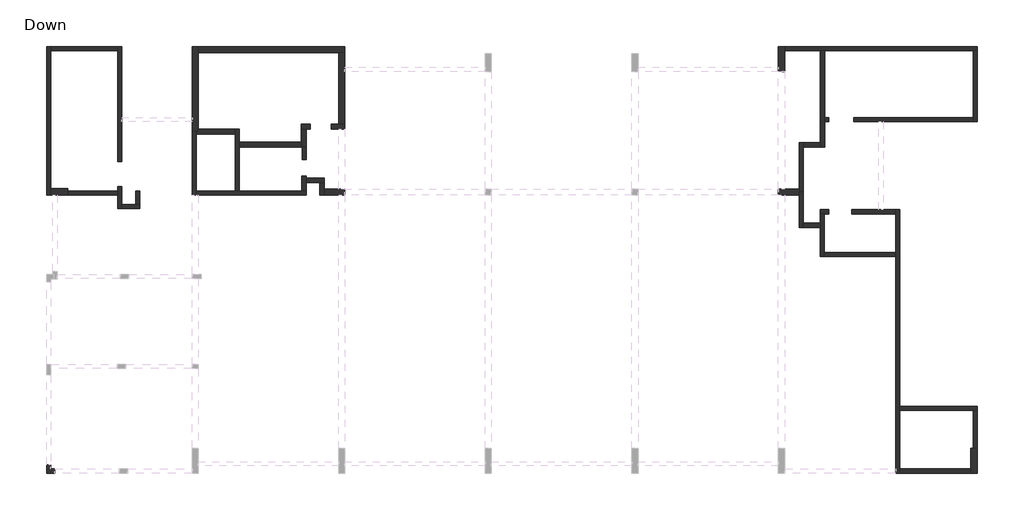
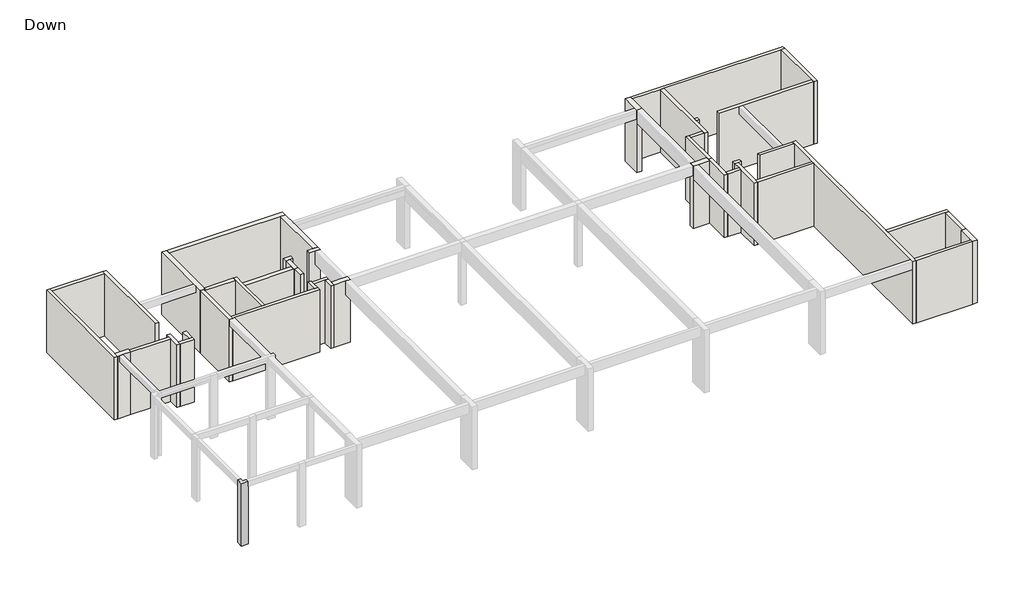
# One storey, part 1 of 2: 44 walls, 1 column.
"""IFC4 building model written with IfcOpenShell, lengths in millimetres."""

from ifc_helpers import new_model, si_unit, origin, origin_with_axes, place, context, project, spatial, polyline, outline, extrude, faceted_brep, element, save

model = new_model("IFC4")

# Units and contexts
model_context = context("Model", 3, world=origin())
ifc_project = project(units=[si_unit("LENGTHUNIT", "METRE", prefix="MILLI")], contexts=[model_context])

# Site, building, storey
site = spatial("IfcSite", under=ifc_project)
building = spatial("IfcBuilding", under=site)
storey = spatial("IfcBuildingStorey", under=building, Name="Down", Elevation=0.0)

# Column
placement = place(None, origin())
element("IfcColumn", 1, ObjectType="L Column : 40/40/20/20", at=placement, inside=storey, context=model_context, shape_type="Brep", body=[
    faceted_brep([(-20892.8250626, 4006.6682295, 0.0), (-20892.8250626, 4406.6682295, 0.0), (-20692.8250626, 4406.6682295, 0.0), (-20692.8250626, 4206.6682295, 0.0), (-20492.8250626, 4206.6682295, 0.0), (-20492.8250626, 4006.6682295, 0.0), (-20892.8250626, 4006.6682295, 4000.0), (-20892.8250626, 4406.6682295, 4000.0), (-20692.8250626, 4406.6682295, 4000.0), (-20692.8250626, 4206.6682295, 4000.0), (-20690.7944112, 4206.6682295, 4000.0), (-20492.8250626, 4206.6682295, 4000.0), (-20492.8250626, 4006.6682295, 4000.0)], [[[0, 1, 2, 3, 4, 5]], [[6, 7, 1, 0]], [[7, 8, 2, 1]], [[8, 9, 3, 2]], [[9, 10, 11, 4, 3]], [[11, 12, 5, 4]], [[12, 6, 0, 5]], [[6, 12, 11, 10, 9, 8, 7]]]),
])

# Walls
element("IfcWall", 2, ObjectType="20", at=placement, inside=storey, context=model_context, shape_type="Brep", body=[
    faceted_brep([(-20890.7944112, 24404.7142065, 0.0), (-20890.7944112, 17304.7716778, 0.0), (-20890.7944112, 17304.7716778, 4000.0), (-20890.7944112, 24404.7142065, 4000.0), (-20690.7944112, 24404.7142065, 0.0), (-20690.7944112, 24404.7142065, 4000.0), (-20690.7944112, 24204.7142065, 4000.0), (-20690.7944112, 19305.3655475, 4000.0), (-20690.7944112, 17605.3655475, 4000.0), (-20690.7944112, 17305.3655475, 4000.0), (-20690.7944112, 17304.7716778, 4000.0), (-20690.7944112, 17304.7716778, 0.0), (-20690.7944112, 17305.3655475, 0.0), (-20690.7944112, 17605.3655475, 0.0), (-20690.7944112, 24204.7142065, 0.0)], [[[0, 1, 2, 3]], [[4, 5, 6, 7, 8, 9, 10, 11, 12, 13, 14]], [[1, 0, 4, 14, 13, 12, 11]], [[2, 1, 11, 10]], [[3, 2, 10, 9, 8, 7, 6, 5]], [[0, 3, 5, 4]]]),
])
element("IfcWall", 3, ObjectType="20", at=placement, inside=storey, context=model_context, shape_type="Brep", body=[
    faceted_brep([(-19891.6373231, 17304.7716778, 0.0), (-17492.1354074, 17304.7716778, 0.0), (-17492.1354074, 17304.7716778, 3790.0), (-17492.1354074, 17304.7716778, 4000.0), (-19891.6373231, 17304.7716778, 4000.0), (-19891.6373231, 17304.7716778, 3790.0), (-19891.6373231, 17504.7716778, 0.0), (-19891.6373231, 17504.7716778, 3790.0), (-19891.6373231, 17504.7716778, 4000.0), (-17492.1354074, 17504.7716778, 4000.0), (-17492.1354074, 17504.7716778, 3790.0), (-17492.1354074, 17504.7716778, 0.0), (-19891.6373231, 17305.3655475, 0.0), (-19891.6373231, 17305.3655475, 4000.0)], [[[0, 1, 2, 3, 4, 5]], [[6, 7, 8, 9, 10, 11]], [[1, 0, 12, 6, 11]], [[4, 3, 9, 8, 13]], [[0, 5, 4, 13, 8, 7, 6, 12]], [[3, 2, 1, 11, 10, 9]]]),
])
element("IfcWall", 4, ObjectType="20", at=placement, inside=storey, context=model_context, shape_type="Brep", body=[
    faceted_brep([(-17492.1354074, 17706.9747429, 0.0), (-17492.1354074, 17504.7716778, 0.0), (-17492.1354074, 17304.7716778, 0.0), (-17492.1354074, 16652.7793406, 0.0), (-17492.1354074, 16652.7793406, 3790.0), (-17492.1354074, 16652.7793406, 4000.0), (-17492.1354074, 17304.7716778, 4000.0), (-17492.1354074, 17504.7716778, 4000.0), (-17492.1354074, 17706.9747429, 4000.0), (-17492.1354074, 17706.9747429, 3790.0), (-17292.1354074, 17706.9747429, 0.0), (-17292.1354074, 17706.9747429, 3790.0), (-17292.1354074, 17706.9747429, 4000.0), (-17292.1354074, 16852.7793406, 4000.0), (-17292.1354074, 16652.7793406, 4000.0), (-17292.1354074, 16652.7793406, 0.0), (-17292.1354074, 16852.7793406, 0.0)], [[[0, 1, 2, 3, 4, 5, 6, 7, 8, 9]], [[10, 11, 12, 13, 14, 15, 16]], [[3, 2, 1, 0, 10, 16, 15]], [[8, 7, 6, 5, 14, 13, 12]], [[0, 9, 8, 12, 11, 10]], [[5, 4, 3, 15, 14]]]),
])
element("IfcWall", 5, ObjectType="20", at=placement, inside=storey, context=model_context, shape_type="Brep", body=[
    faceted_brep([(-17292.1354074, 18905.1165054, 0.0), (-17292.1354074, 24404.7142065, 0.0), (-17292.1354074, 24404.7142065, 4000.0), (-17292.1354074, 20806.0552027, 4000.0), (-17292.1354074, 18905.1165054, 4000.0), (-17292.1354074, 18905.1165054, 3790.0), (-17492.1354074, 18905.1165054, 0.0), (-17492.1354074, 18905.1165054, 3790.0), (-17492.1354074, 18905.1165054, 4000.0), (-17492.1354074, 19305.3655475, 4000.0), (-17492.1354074, 24204.7142065, 4000.0), (-17492.1354074, 24404.7142065, 4000.0), (-17492.1354074, 24404.7142065, 0.0), (-17492.1354074, 24204.7142065, 0.0)], [[[0, 1, 2, 3, 4, 5]], [[6, 7, 8, 9, 10, 11, 12, 13]], [[1, 0, 6, 13, 12]], [[4, 3, 2, 11, 10, 9, 8]], [[0, 5, 4, 8, 7, 6]], [[2, 1, 12, 11]]]),
])
element("IfcWall", 6, ObjectType="20", at=placement, inside=storey, context=model_context, shape_type="SweptSolid", body=[
    extrude(outline(polyline([(-20690.7944112, 24404.7142065), (-17492.1354074, 24404.7142065), (-17492.1354074, 24204.7142065), (-20690.7944112, 24204.7142065), (-20690.7944112, 24404.7142065)])), origin_with_axes(), (0.0, 0.0, 1.0), 4000.0),
])
element("IfcWall", 7, ObjectType="20", at=placement, inside=storey, context=model_context, shape_type="Brep", body=[
    faceted_brep([(-17292.1354074, 16652.7793406, 0.0), (-16441.1583959, 16652.7793406, 0.0), (-16441.1583959, 16652.7793406, 3790.0), (-16441.1583959, 16652.7793406, 4000.0), (-17292.1354074, 16652.7793406, 4000.0), (-17292.1354074, 16852.7793406, 0.0), (-17292.1354074, 16852.7793406, 3790.0), (-17292.1354074, 16852.7793406, 4000.0), (-16641.1583959, 16852.7793406, 4000.0), (-16441.1583959, 16852.7793406, 4000.0), (-16441.1583959, 16852.7793406, 0.0), (-16641.1583959, 16852.7793406, 0.0)], [[[0, 1, 2, 3, 4]], [[5, 6, 7, 8, 9, 10, 11]], [[1, 0, 5, 11, 10]], [[4, 3, 9, 8, 7]], [[0, 4, 7, 6, 5]], [[3, 2, 1, 10, 9]]]),
])
element("IfcWall", 8, ObjectType="20", at=placement, inside=storey, context=model_context, shape_type="Brep", body=[
    faceted_brep([(-16441.1583959, 16852.7793406, 0.0), (-16441.1583959, 17503.7563521, 0.0), (-16441.1583959, 17503.7563521, 3790.0), (-16441.1583959, 17503.7563521, 4000.0), (-16441.1583959, 16852.7793406, 4000.0), (-16641.1583959, 16852.7793406, 0.0), (-16641.1583959, 16852.7793406, 3790.0), (-16641.1583959, 16852.7793406, 4000.0), (-16641.1583959, 17503.7563521, 4000.0), (-16641.1583959, 17503.7563521, 3790.0), (-16641.1583959, 17503.7563521, 0.0)], [[[0, 1, 2, 3, 4]], [[5, 6, 7, 8, 9, 10]], [[1, 0, 5, 10]], [[3, 2, 1, 10, 9, 8]], [[4, 3, 8, 7]], [[0, 4, 7, 6, 5]]]),
])
element("IfcWall", 9, ObjectType="20", at=placement, inside=storey, context=model_context, shape_type="Brep", body=[
    faceted_brep([(-11890.9285108, 20459.7142065, 0.0), (-11890.9285108, 20209.7142065, 0.0), (-11890.9285108, 17504.7716778, 0.0), (-11890.9285108, 17504.7716778, 4000.0), (-11890.9285108, 20209.7142065, 4000.0), (-11890.9285108, 20459.7142065, 4000.0), (-11690.9285108, 20459.7142065, 0.0), (-11690.9285108, 20459.7142065, 3790.0), (-11690.9285108, 20459.7142065, 4000.0), (-11690.9285108, 19844.6567352, 4000.0), (-11690.9285108, 19594.6567352, 4000.0), (-11690.9285108, 17504.7716778, 4000.0), (-11690.9285108, 17504.7716778, 3790.0), (-11690.9285108, 17504.7716778, 0.0), (-11690.9285108, 19594.6567352, 0.0), (-11690.9285108, 19844.6567352, 0.0)], [[[0, 1, 2, 3, 4, 5]], [[6, 7, 8, 9, 10, 11, 12, 13, 14, 15]], [[2, 1, 0, 6, 15, 14, 13]], [[5, 4, 3, 11, 10, 9, 8]], [[3, 2, 13, 12, 11]], [[0, 5, 8, 7, 6]]]),
])
element("IfcWall", 10, ObjectType="20", at=placement, inside=storey, context=model_context, shape_type="Brep", body=[
    faceted_brep([(-13743.2656756, 17304.7716778, 0.0), (-8494.4725721, 17304.7716778, 0.0), (-8494.4725721, 17304.7716778, 3790.0), (-8494.4725721, 17304.7716778, 4000.0), (-13643.2656756, 17304.7716778, 4000.0), (-13743.2656756, 17304.7716778, 4000.0), (-13743.2656756, 17504.7716778, 0.0), (-13743.2656756, 17504.7716778, 4000.0), (-11890.9285108, 17504.7716778, 4000.0), (-11690.9285108, 17504.7716778, 4000.0), (-8694.4725721, 17504.7716778, 4000.0), (-8494.4725721, 17504.7716778, 4000.0), (-8494.4725721, 17504.7716778, 0.0), (-8694.4725721, 17504.7716778, 0.0), (-11690.9285108, 17504.7716778, 0.0), (-11890.9285108, 17504.7716778, 0.0)], [[[0, 1, 2, 3, 4, 5]], [[6, 7, 8, 9, 10, 11, 12, 13, 14, 15]], [[1, 0, 6, 15, 14, 13, 12]], [[5, 4, 3, 11, 10, 9, 8, 7]], [[3, 2, 1, 12, 11]], [[0, 5, 7, 6]]]),
])
element("IfcWall", 11, ObjectType="20", at=placement, inside=storey, context=model_context, shape_type="Brep", body=[
    faceted_brep([(-8494.4725721, 17504.7716778, 0.0), (-8494.4725721, 17905.9594172, 0.0), (-8494.4725721, 18105.9594172, 0.0), (-8494.4725721, 18206.553287, 0.0), (-8494.4725721, 18206.553287, 3790.0), (-8494.4725721, 18206.553287, 4000.0), (-8494.4725721, 18105.9594172, 4000.0), (-8494.4725721, 17905.9594172, 4000.0), (-8494.4725721, 17504.7716778, 4000.0), (-8694.4725721, 17504.7716778, 0.0), (-8694.4725721, 17504.7716778, 3790.0), (-8694.4725721, 17504.7716778, 4000.0), (-8694.4725721, 18206.553287, 4000.0), (-8694.4725721, 18206.553287, 3790.0), (-8694.4725721, 18206.553287, 0.0)], [[[0, 1, 2, 3, 4, 5, 6, 7, 8]], [[9, 10, 11, 12, 13, 14]], [[3, 2, 1, 0, 9, 14]], [[5, 4, 3, 14, 13, 12]], [[8, 7, 6, 5, 12, 11]], [[0, 8, 11, 10, 9]]]),
])
element("IfcWall", 12, ObjectType="20", at=placement, inside=storey, context=model_context, shape_type="Brep", body=[
    faceted_brep([(-8485.7944112, 19006.7257008, 0.0), (-8485.7944112, 19594.6567352, 0.0), (-8485.7944112, 19594.6567352, 4000.0), (-8485.7944112, 19006.7257008, 4000.0), (-8485.7944112, 19006.7257008, 3790.0), (-8685.7944112, 19006.7257008, 0.0), (-8685.7944112, 19006.7257008, 3790.0), (-8685.7944112, 19006.7257008, 4000.0), (-8685.7944112, 19594.6567352, 4000.0), (-8685.7944112, 19594.6567352, 3790.0), (-8685.7944112, 19594.6567352, 0.0)], [[[0, 1, 2, 3, 4]], [[5, 6, 7, 8, 9, 10]], [[1, 0, 5, 10]], [[3, 2, 8, 7]], [[0, 4, 3, 7, 6, 5]], [[2, 1, 10, 9, 8]]]),
])
element("IfcWall", 13, ObjectType="20", at=placement, inside=storey, context=model_context, shape_type="Brep", body=[
    faceted_brep([(-13943.2656756, 20334.7142065, 0.0), (-13943.2656756, 17304.7716778, 0.0), (-13943.2656756, 17304.7716778, 3600.0), (-13943.2656756, 17304.7716778, 4000.0), (-13943.2656756, 20334.7142065, 4000.0), (-13743.2656756, 20334.7142065, 0.0), (-13743.2656756, 20334.7142065, 4000.0), (-13743.2656756, 20209.7142065, 4000.0), (-13743.2656756, 17504.7716778, 4000.0), (-13743.2656756, 17304.7716778, 4000.0), (-13743.2656756, 17304.7716778, 0.0), (-13743.2656756, 17504.7716778, 0.0), (-13743.2656756, 20209.7142065, 0.0)], [[[0, 1, 2, 3, 4]], [[5, 6, 7, 8, 9, 10, 11, 12]], [[1, 0, 5, 12, 11, 10]], [[4, 3, 9, 8, 7, 6]], [[0, 4, 6, 5]], [[3, 2, 1, 10, 9]]]),
])
element("IfcWall", 14, ObjectType="20", at=placement, inside=storey, context=model_context, shape_type="Brep", body=[
    faceted_brep([(-8494.4725721, 17905.9594172, 0.0), (-7834.4725721, 17905.9594172, 0.0), (-7634.4725721, 17905.9594172, 0.0), (-7634.4725721, 17905.9594172, 4000.0), (-7834.4725721, 17905.9594172, 4000.0), (-8494.4725721, 17905.9594172, 4000.0), (-8494.4725721, 17905.9594172, 3790.0), (-8494.4725721, 18105.9594172, 0.0), (-8494.4725721, 18105.9594172, 3790.0), (-8494.4725721, 18105.9594172, 4000.0), (-7634.4725721, 18105.9594172, 4000.0), (-7634.4725721, 18105.9594172, 3790.0), (-7634.4725721, 18105.9594172, 0.0)], [[[0, 1, 2, 3, 4, 5, 6]], [[7, 8, 9, 10, 11, 12]], [[2, 1, 0, 7, 12]], [[5, 4, 3, 10, 9]], [[0, 6, 5, 9, 8, 7]], [[3, 2, 12, 11, 10]]]),
])
element("IfcWall", 15, ObjectType="20", at=placement, inside=storey, context=model_context, shape_type="Brep", body=[
    faceted_brep([(-7834.4725721, 17905.9594172, 0.0), (-7834.4725721, 17297.4228975, 0.0), (-7834.4725721, 17297.4228975, 3790.0), (-7834.4725721, 17297.4228975, 4000.0), (-7834.4725721, 17905.9594172, 4000.0), (-7834.4725721, 17905.9594172, 3790.0), (-7634.4725721, 17905.9594172, 0.0), (-7634.4725721, 17905.9594172, 4000.0), (-7634.4725721, 17597.4228975, 4000.0), (-7634.4725721, 17297.4228975, 4000.0), (-7634.4725721, 17297.4228975, 0.0), (-7634.4725721, 17597.4228975, 0.0)], [[[0, 1, 2, 3, 4, 5]], [[6, 7, 8, 9, 10, 11]], [[1, 0, 6, 11, 10]], [[4, 3, 9, 8, 7]], [[0, 5, 4, 7, 6]], [[3, 2, 1, 10, 9]]]),
])
element("IfcWall", 16, ObjectType="20", at=placement, inside=storey, context=model_context, shape_type="Brep", body=[
    faceted_brep([(14358.5350907, 24204.7142065, 0.0), (16064.3013742, 24204.7142065, 0.0), (16264.3013742, 24204.7142065, 0.0), (23368.5350907, 24204.7142065, 0.0), (23568.5350907, 24204.7142065, 0.0), (23568.5350907, 24204.7142065, 4000.0), (23368.5350907, 24204.7142065, 4000.0), (18304.3013742, 24204.7142065, 4000.0), (16264.3013742, 24204.7142065, 4000.0), (16064.3013742, 24204.7142065, 4000.0), (14358.5350907, 24204.7142065, 4000.0), (14358.5350907, 24204.7142065, 3790.0), (14358.5350907, 24404.7142065, 0.0), (14358.5350907, 24404.7142065, 4000.0), (23568.5350907, 24404.7142065, 4000.0), (23568.5350907, 24404.7142065, 0.0)], [[[0, 1, 2, 3, 4, 5, 6, 7, 8, 9, 10, 11]], [[12, 13, 14, 15]], [[4, 3, 2, 1, 0, 12, 15]], [[10, 9, 8, 7, 6, 5, 14, 13]], [[0, 11, 10, 13, 12]], [[5, 4, 15, 14]]]),
])
element("IfcWall", 17, ObjectType="20", at=placement, inside=storey, context=model_context, shape_type="Brep", body=[
    faceted_brep([(23368.5350907, 24204.7142065, 0.0), (23368.5350907, 21004.7142065, 0.0), (23368.5350907, 20804.7142065, 0.0), (23368.5350907, 20804.7142065, 4000.0), (23368.5350907, 21004.7142065, 4000.0), (23368.5350907, 24204.7142065, 4000.0), (23568.5350907, 24204.7142065, 0.0), (23568.5350907, 24204.7142065, 4000.0), (23568.5350907, 20804.7142065, 4000.0), (23568.5350907, 20804.7142065, 0.0)], [[[0, 1, 2, 3, 4, 5]], [[6, 7, 8, 9]], [[2, 1, 0, 6, 9]], [[5, 4, 3, 8, 7]], [[0, 5, 7, 6]], [[3, 2, 9, 8]]]),
])
element("IfcWall", 18, ObjectType="20", at=placement, inside=storey, context=model_context, shape_type="Brep", body=[
    faceted_brep([(23368.5350907, 21004.7142065, 0.0), (17668.5350907, 21004.7142065, 0.0), (17668.5350907, 21004.7142065, 3790.0), (17668.5350907, 21004.7142065, 4000.0), (18304.3013742, 21004.7142065, 4000.0), (23368.5350907, 21004.7142065, 4000.0), (23368.5350907, 20804.7142065, 0.0), (23368.5350907, 20804.7142065, 4000.0), (17668.5350907, 20804.7142065, 4000.0), (17668.5350907, 20804.7142065, 3790.0), (17668.5350907, 20804.7142065, 0.0)], [[[0, 1, 2, 3, 4, 5]], [[6, 7, 8, 9, 10]], [[1, 0, 6, 10]], [[3, 2, 1, 10, 9, 8]], [[5, 4, 3, 8, 7]], [[0, 5, 7, 6]]]),
])
element("IfcWall", 19, ObjectType="20", at=placement, inside=storey, context=model_context, shape_type="Brep", body=[
    faceted_brep([(16459.0523321, 21006.0552027, 0.0), (16264.3013742, 21006.0552027, 0.0), (16264.3013742, 21006.0552027, 3790.0), (16264.3013742, 21006.0552027, 4000.0), (16459.0523321, 21006.0552027, 4000.0), (16459.0523321, 21006.0552027, 3790.0), (16459.0523321, 20806.0552027, 0.0), (16459.0523321, 20806.0552027, 4000.0), (16264.3013742, 20806.0552027, 4000.0), (16264.3013742, 20806.0552027, 0.0)], [[[0, 1, 2, 3, 4, 5]], [[6, 7, 8, 9]], [[1, 0, 6, 9]], [[4, 3, 8, 7]], [[0, 5, 4, 7, 6]], [[3, 2, 1, 9, 8]]]),
])
element("IfcWall", 20, ObjectType="20", at=placement, inside=storey, context=model_context, shape_type="Brep", body=[
    faceted_brep([(16064.3013742, 24204.7142065, 0.0), (16064.3013742, 19803.6797237, 0.0), (16064.3013742, 19603.6797237, 0.0), (16064.3013742, 19603.6797237, 4000.0), (16064.3013742, 19803.6797237, 4000.0), (16064.3013742, 24204.7142065, 4000.0), (16064.3013742, 24204.7142065, 3790.0), (16264.3013742, 24204.7142065, 0.0), (16264.3013742, 24204.7142065, 3790.0), (16264.3013742, 24204.7142065, 4000.0), (16264.3013742, 21006.0552027, 4000.0), (16264.3013742, 20806.0552027, 4000.0), (16264.3013742, 19603.6797237, 4000.0), (16264.3013742, 19603.6797237, 0.0), (16264.3013742, 20806.0552027, 0.0), (16264.3013742, 21006.0552027, 0.0)], [[[0, 1, 2, 3, 4, 5, 6]], [[7, 8, 9, 10, 11, 12, 13, 14, 15]], [[2, 1, 0, 7, 15, 14, 13]], [[5, 4, 3, 12, 11, 10, 9]], [[0, 6, 5, 9, 8, 7]], [[3, 2, 13, 12]]]),
])
element("IfcWall", 21, ObjectType="20", at=placement, inside=storey, context=model_context, shape_type="Brep", body=[
    faceted_brep([(16064.3013742, 19803.6797237, 0.0), (15257.6921788, 19803.6797237, 0.0), (15257.6921788, 19803.6797237, 4000.0), (16064.3013742, 19803.6797237, 4000.0), (16064.3013742, 19803.6797237, 3790.0), (16064.3013742, 19603.6797237, 0.0), (16064.3013742, 19603.6797237, 4000.0), (15257.6921788, 19603.6797237, 4000.0), (15257.6921788, 19603.6797237, 0.0)], [[[0, 1, 2, 3, 4]], [[5, 6, 7, 8]], [[1, 0, 5, 8]], [[3, 2, 7, 6]], [[0, 4, 3, 6, 5]], [[2, 1, 8, 7]]]),
])
element("IfcWall", 22, ObjectType="20", at=placement, inside=storey, context=model_context, shape_type="Brep", body=[
    faceted_brep([(15057.6921788, 19803.6797237, 0.0), (15057.6921788, 17597.4228975, 0.0), (15057.6921788, 17447.4228975, 0.0), (15057.6921788, 17447.4228975, 4000.0), (15057.6921788, 17597.4228975, 4000.0), (15057.6921788, 19803.6797237, 4000.0), (15057.6921788, 19803.6797237, 3790.0), (15257.6921788, 19803.6797237, 0.0), (15257.6921788, 19803.6797237, 4000.0), (15257.6921788, 19603.6797237, 4000.0), (15257.6921788, 17447.4228975, 4000.0), (15257.6921788, 17447.4228975, 0.0), (15257.6921788, 19603.6797237, 0.0)], [[[0, 1, 2, 3, 4, 5, 6]], [[7, 8, 9, 10, 11, 12]], [[2, 1, 0, 7, 12, 11]], [[3, 2, 11, 10]], [[5, 4, 3, 10, 9, 8]], [[0, 6, 5, 8, 7]]]),
])
element("IfcWall", 23, ObjectType="20", at=placement, inside=storey, context=model_context, shape_type="Brep", body=[
    faceted_brep([(15257.6921788, 15755.2314479, 0.0), (15257.6921788, 15955.2314479, 0.0), (15257.6921788, 17447.4228975, 0.0), (15257.6921788, 17447.4228975, 4000.0), (15257.6921788, 15955.2314479, 4000.0), (15257.6921788, 15755.2314479, 4000.0), (15057.6921788, 15755.2314479, 0.0), (15057.6921788, 15755.2314479, 3790.0), (15057.6921788, 15755.2314479, 4000.0), (15057.6921788, 17297.4228975, 4000.0), (15057.6921788, 17447.4228975, 4000.0), (15057.6921788, 17447.4228975, 0.0), (15057.6921788, 17297.4228975, 0.0)], [[[0, 1, 2, 3, 4, 5]], [[6, 7, 8, 9, 10, 11, 12]], [[2, 1, 0, 6, 12, 11]], [[3, 2, 11, 10]], [[5, 4, 3, 10, 9, 8]], [[0, 5, 8, 7, 6]]]),
])
element("IfcWall", 24, ObjectType="20", at=placement, inside=storey, context=model_context, shape_type="Brep", body=[
    faceted_brep([(15257.6921788, 15755.2314479, 0.0), (16056.849267, 15755.2314479, 0.0), (16056.849267, 15755.2314479, 3790.0), (16056.849267, 15755.2314479, 4000.0), (15257.6921788, 15755.2314479, 4000.0), (15257.6921788, 15955.2314479, 0.0), (15257.6921788, 15955.2314479, 4000.0), (16056.849267, 15955.2314479, 4000.0), (16056.849267, 15955.2314479, 0.0)], [[[0, 1, 2, 3, 4]], [[5, 6, 7, 8]], [[1, 0, 5, 8]], [[4, 3, 7, 6]], [[0, 4, 6, 5]], [[3, 2, 1, 8, 7]]]),
])
element("IfcWall", 25, ObjectType="20", at=placement, inside=storey, context=model_context, shape_type="Brep", body=[
    faceted_brep([(16056.849267, 16406.2084594, 0.0), (16056.849267, 15955.2314479, 0.0), (16056.849267, 15755.2314479, 0.0), (16056.849267, 14353.8712946, 0.0), (16056.849267, 14353.8712946, 3790.0), (16056.849267, 14353.8712946, 4000.0), (16056.849267, 15755.2314479, 4000.0), (16056.849267, 15955.2314479, 4000.0), (16056.849267, 16406.2084594, 4000.0), (16256.849267, 16406.2084594, 0.0), (16256.849267, 16406.2084594, 4000.0), (16256.849267, 14553.8712946, 4000.0), (16256.849267, 14353.8712946, 4000.0), (16256.849267, 14353.8712946, 0.0), (16256.849267, 14553.8712946, 0.0)], [[[0, 1, 2, 3, 4, 5, 6, 7, 8]], [[9, 10, 11, 12, 13, 14]], [[3, 2, 1, 0, 9, 14, 13]], [[8, 7, 6, 5, 12, 11, 10]], [[5, 4, 3, 13, 12]], [[0, 8, 10, 9]]]),
])
element("IfcWall", 26, ObjectType="20", at=placement, inside=storey, context=model_context, shape_type="Brep", body=[
    faceted_brep([(16256.849267, 14353.8712946, 0.0), (19658.7266616, 14353.8712946, 0.0), (19658.7266616, 14353.8712946, 3790.0), (19658.7266616, 14353.8712946, 4000.0), (16256.849267, 14353.8712946, 4000.0), (16256.849267, 14553.8712946, 0.0), (16256.849267, 14553.8712946, 4000.0), (19658.7266616, 14553.8712946, 4000.0), (19658.7266616, 14553.8712946, 0.0)], [[[0, 1, 2, 3, 4]], [[5, 6, 7, 8]], [[1, 0, 5, 8]], [[4, 3, 7, 6]], [[0, 4, 6, 5]], [[3, 2, 1, 8, 7]]]),
])
element("IfcWall", 27, ObjectType="20", at=placement, inside=storey, context=model_context, shape_type="Brep", body=[
    faceted_brep([(19658.7266616, 16606.2084594, 0.0), (19658.7266616, 16406.2084594, 0.0), (19658.7266616, 14553.8712946, 0.0), (19658.7266616, 14353.8712946, 0.0), (19658.7266616, 4004.8099919, 0.0), (19658.7266616, 4004.8099919, 3500.0), (19658.7266616, 4004.8099919, 4000.0), (19658.7266616, 4204.8099919, 4000.0), (19658.7266616, 14353.8712946, 4000.0), (19658.7266616, 14553.8712946, 4000.0), (19658.7266616, 16406.2084594, 4000.0), (19658.7266616, 16606.2084594, 4000.0), (19858.7266616, 16606.2084594, 0.0), (19858.7266616, 16606.2084594, 4000.0), (19858.7266616, 7204.1394939, 4000.0), (19858.7266616, 7004.1394939, 4000.0), (19858.7266616, 4204.8099919, 4000.0), (19858.7266616, 4004.8099919, 4000.0), (19858.7266616, 4004.8099919, 0.0), (19858.7266616, 4204.8099919, 0.0), (19858.7266616, 7004.1394939, 0.0), (19858.7266616, 7204.1394939, 0.0)], [[[0, 1, 2, 3, 4, 5, 6, 7, 8, 9, 10, 11]], [[12, 13, 14, 15, 16, 17, 18, 19, 20, 21]], [[4, 3, 2, 1, 0, 12, 21, 20, 19, 18]], [[11, 10, 9, 8, 7, 6, 17, 16, 15, 14, 13]], [[0, 11, 13, 12]], [[6, 5, 4, 18, 17]]]),
])
element("IfcWall", 28, ObjectType="20", at=placement, inside=storey, context=model_context, shape_type="SweptSolid", body=[
    extrude(outline(polyline([(17559.8186156, 16606.2084594), (19658.7266616, 16606.2084594), (19658.7266616, 16406.2084594), (17559.8186156, 16406.2084594), (17559.8186156, 16606.2084594)])), origin_with_axes(), (0.0, 0.0, 1.0), 4000.0),
])
element("IfcWall", 29, ObjectType="20", at=placement, inside=storey, context=model_context, shape_type="Brep", body=[
    faceted_brep([(16459.0523321, 16606.2084594, 0.0), (16056.849267, 16606.2084594, 0.0), (16056.849267, 16606.2084594, 4000.0), (16459.0523321, 16606.2084594, 4000.0), (16459.0523321, 16406.2084594, 0.0), (16459.0523321, 16406.2084594, 4000.0), (16256.849267, 16406.2084594, 4000.0), (16056.849267, 16406.2084594, 4000.0), (16056.849267, 16406.2084594, 0.0), (16256.849267, 16406.2084594, 0.0)], [[[0, 1, 2, 3]], [[4, 5, 6, 7, 8, 9]], [[1, 0, 4, 9, 8]], [[3, 2, 7, 6, 5]], [[0, 3, 5, 4]], [[2, 1, 8, 7]]]),
])
element("IfcWall", 30, ObjectType="20", at=placement, inside=storey, context=model_context, shape_type="Brep", body=[
    faceted_brep([(19858.7266616, 7004.1394939, 0.0), (23358.9948608, 7004.1394939, 0.0), (23558.9948608, 7004.1394939, 0.0), (23558.9948608, 7004.1394939, 4000.0), (23358.9948608, 7004.1394939, 4000.0), (19858.7266616, 7004.1394939, 4000.0), (19858.7266616, 7004.1394939, 3790.0), (19858.7266616, 7204.1394939, 0.0), (19858.7266616, 7204.1394939, 4000.0), (23558.9948608, 7204.1394939, 4000.0), (23558.9948608, 7204.1394939, 0.0)], [[[0, 1, 2, 3, 4, 5, 6]], [[7, 8, 9, 10]], [[2, 1, 0, 7, 10]], [[5, 4, 3, 9, 8]], [[0, 6, 5, 8, 7]], [[3, 2, 10, 9]]]),
])
element("IfcWall", 31, ObjectType="20", at=placement, inside=storey, context=model_context, shape_type="Brep", body=[
    faceted_brep([(23358.9948608, 7004.1394939, 0.0), (23358.9948608, 5204.1394939, 0.0), (23358.9948608, 5204.1394939, 3790.0), (23358.9948608, 5204.1394939, 4000.0), (23358.9948608, 7004.1394939, 4000.0), (23358.9948608, 7004.1394939, 3790.0), (23558.9948608, 7004.1394939, 0.0), (23558.9948608, 7004.1394939, 4000.0), (23558.9948608, 5204.1394939, 4000.0), (23558.9948608, 5204.1394939, 0.0)], [[[0, 1, 2, 3, 4, 5]], [[6, 7, 8, 9]], [[1, 0, 6, 9]], [[3, 2, 1, 9, 8]], [[4, 3, 8, 7]], [[0, 5, 4, 7, 6]]]),
])
element("IfcWall", 32, ObjectType="20", at=placement, inside=storey, context=model_context, shape_type="Brep", body=[
    faceted_brep([(23258.9948608, 4204.8099919, 0.0), (19858.7266616, 4204.8099919, 0.0), (19858.7266616, 4204.8099919, 3790.0), (19858.7266616, 4204.8099919, 4000.0), (23258.9948608, 4204.8099919, 4000.0), (23258.9948608, 4204.8099919, 3790.0), (23258.9948608, 4004.8099919, 0.0), (23258.9948608, 4004.8099919, 4000.0), (19858.7266616, 4004.8099919, 4000.0), (19858.7266616, 4004.8099919, 0.0)], [[[0, 1, 2, 3, 4, 5]], [[6, 7, 8, 9]], [[1, 0, 6, 9]], [[4, 3, 8, 7]], [[0, 5, 4, 7, 6]], [[3, 2, 1, 9, 8]]]),
])
element("IfcWall", 33, ObjectType="25", at=placement, inside=storey, context=model_context, shape_type="Brep", body=[
    faceted_brep([(-6644.3384725, 20704.6567352, 0.0), (-6944.3384725, 20704.6567352, 0.0), (-7292.0970932, 20704.6567352, 0.0), (-7292.0970932, 20704.6567352, 3790.0), (-7292.0970932, 20704.6567352, 4000.0), (-6944.3384725, 20704.6567352, 4000.0), (-6644.3384725, 20704.6567352, 4000.0), (-6644.3384725, 20454.6567352, 0.0), (-6644.3384725, 20454.6567352, 3150.0), (-6644.3384725, 20454.6567352, 3790.0), (-6644.3384725, 20454.6567352, 4000.0), (-6674.3384725, 20454.6567352, 4000.0), (-6944.3384725, 20454.6567352, 4000.0), (-7292.0970932, 20454.6567352, 4000.0), (-7292.0970932, 20454.6567352, 3790.0), (-7292.0970932, 20454.6567352, 0.0)], [[[0, 1, 2, 3, 4, 5, 6]], [[7, 8, 9, 10, 11, 12, 13, 14, 15]], [[2, 1, 0, 7, 15]], [[4, 3, 2, 15, 14, 13]], [[6, 5, 4, 13, 12, 11, 10]], [[0, 6, 10, 9, 8, 7]]]),
])
element("IfcWall", 34, ObjectType="25", at=placement, inside=storey, context=model_context, shape_type="Brep", body=[
    faceted_brep([(-8291.2541813, 20704.6567352, 0.0), (-8735.7944112, 20704.6567352, 0.0), (-8735.7944112, 20704.6567352, 3790.0), (-8735.7944112, 20704.6567352, 4000.0), (-8291.2541813, 20704.6567352, 4000.0), (-8291.2541813, 20704.6567352, 3790.0), (-8291.2541813, 20454.6567352, 0.0), (-8291.2541813, 20454.6567352, 3790.0), (-8291.2541813, 20454.6567352, 4000.0), (-8485.7944112, 20454.6567352, 4000.0), (-8735.7944112, 20454.6567352, 4000.0), (-8735.7944112, 20454.6567352, 0.0), (-8485.7944112, 20454.6567352, 0.0)], [[[0, 1, 2, 3, 4, 5]], [[6, 7, 8, 9, 10, 11, 12]], [[1, 0, 6, 12, 11]], [[4, 3, 10, 9, 8]], [[0, 5, 4, 8, 7, 6]], [[3, 2, 1, 11, 10]]]),
])
element("IfcWall", 35, ObjectType="25", at=placement, inside=storey, context=model_context, shape_type="Brep", body=[
    faceted_brep([(-8735.7944112, 20454.6567352, 0.0), (-8735.7944112, 19844.6567352, 0.0), (-8735.7944112, 19594.6567352, 0.0), (-8735.7944112, 19594.6567352, 4000.0), (-8735.7944112, 19844.6567352, 4000.0), (-8735.7944112, 20454.6567352, 4000.0), (-8485.7944112, 20454.6567352, 0.0), (-8485.7944112, 20454.6567352, 3790.0), (-8485.7944112, 20454.6567352, 4000.0), (-8485.7944112, 19594.6567352, 4000.0), (-8485.7944112, 19594.6567352, 0.0), (-8685.7944112, 19594.6567352, 0.0), (-8685.7944112, 19594.6567352, 4000.0)], [[[0, 1, 2, 3, 4, 5]], [[6, 7, 8, 9, 10]], [[2, 1, 0, 6, 10, 11]], [[5, 4, 3, 12, 9, 8]], [[0, 5, 8, 7, 6]], [[3, 2, 11, 10, 9, 12]]]),
])
element("IfcWall", 36, ObjectType="25", at=placement, inside=storey, context=model_context, shape_type="Brep", body=[
    faceted_brep([(-8735.7944112, 19844.6567352, 0.0), (-11690.9285108, 19844.6567352, 0.0), (-11690.9285108, 19844.6567352, 3790.0), (-11690.9285108, 19844.6567352, 4000.0), (-8735.7944112, 19844.6567352, 4000.0), (-8735.7944112, 19844.6567352, 3790.0), (-8735.7944112, 19594.6567352, 0.0), (-8735.7944112, 19594.6567352, 4000.0), (-11690.9285108, 19594.6567352, 4000.0), (-11690.9285108, 19594.6567352, 3790.0), (-11690.9285108, 19594.6567352, 0.0)], [[[0, 1, 2, 3, 4, 5]], [[6, 7, 8, 9, 10]], [[1, 0, 6, 10]], [[4, 3, 8, 7]], [[0, 5, 4, 7, 6]], [[3, 2, 1, 10, 9, 8]]]),
])
element("IfcWall", 37, ObjectType="25", at=placement, inside=storey, context=model_context, shape_type="Brep", body=[
    faceted_brep([(-11890.9285108, 20459.7142065, 0.0), (-13643.2656756, 20459.7142065, 0.0), (-13643.2656756, 20459.7142065, 3790.0), (-13643.2656756, 20459.7142065, 4000.0), (-11890.9285108, 20459.7142065, 4000.0), (-11890.9285108, 20209.7142065, 0.0), (-11890.9285108, 20209.7142065, 4000.0), (-13743.2656756, 20209.7142065, 4000.0), (-13743.2656756, 20209.7142065, 0.0), (-13743.2656756, 20334.7142065, 0.0), (-13643.2656756, 20334.7142065, 0.0), (-13643.2656756, 20334.7142065, 4000.0), (-13743.2656756, 20334.7142065, 4000.0)], [[[0, 1, 2, 3, 4]], [[5, 6, 7, 8]], [[1, 0, 5, 8, 9, 10]], [[4, 3, 11, 12, 7, 6]], [[0, 4, 6, 5]], [[3, 2, 1, 10, 11]], [[10, 9, 12, 11]], [[9, 8, 7, 12]]]),
])
element("IfcWall", 38, ObjectType="30", at=placement, inside=storey, context=model_context, shape_type="Brep", body=[
    faceted_brep([(-19891.6373231, 17605.3655475, 0.0), (-20690.7944112, 17605.3655475, 0.0), (-20690.7944112, 17605.3655475, 3790.0), (-20690.7944112, 17605.3655475, 4000.0), (-19891.6373231, 17605.3655475, 4000.0), (-19891.6373231, 17605.3655475, 3790.0), (-19891.6373231, 17305.3655475, 0.0), (-19891.6373231, 17305.3655475, 3790.0), (-19891.6373231, 17305.3655475, 4000.0), (-20386.1465057, 17305.3655475, 4000.0), (-20690.7944112, 17305.3655475, 4000.0), (-20690.7944112, 17305.3655475, 0.0), (-19891.6373231, 17504.7716778, 0.0), (-19891.6373231, 17504.7716778, 4000.0)], [[[0, 1, 2, 3, 4, 5]], [[6, 7, 8, 9, 10, 11]], [[1, 0, 12, 6, 11]], [[4, 3, 10, 9, 8, 13]], [[0, 5, 4, 13, 8, 7, 6, 12]], [[3, 2, 1, 11, 10]]]),
])
element("IfcWall", 39, ObjectType="30", at=placement, inside=storey, context=model_context, shape_type="Brep", body=[
    faceted_brep([(-13943.2656756, 24404.7142065, 0.0), (-13943.2656756, 20334.7142065, 0.0), (-13943.2656756, 20334.7142065, 4000.0), (-13943.2656756, 20806.0552027, 4000.0), (-13943.2656756, 24404.7142065, 4000.0), (-13643.2656756, 24404.7142065, 0.0), (-13643.2656756, 24404.7142065, 4000.0), (-13643.2656756, 24104.7142065, 4000.0), (-13643.2656756, 20459.7142065, 4000.0), (-13643.2656756, 20334.7142065, 4000.0), (-13643.2656756, 20334.7142065, 0.0), (-13643.2656756, 20459.7142065, 0.0), (-13643.2656756, 24104.7142065, 0.0), (-13743.2656756, 20334.7142065, 0.0), (-13743.2656756, 20334.7142065, 4000.0)], [[[0, 1, 2, 3, 4]], [[5, 6, 7, 8, 9, 10, 11, 12]], [[1, 0, 5, 12, 11, 10, 13]], [[2, 1, 13, 10, 9, 14]], [[4, 3, 2, 14, 9, 8, 7, 6]], [[0, 4, 6, 5]]]),
])
element("IfcWall", 40, ObjectType="30", at=placement, inside=storey, context=model_context, shape_type="Brep", body=[
    faceted_brep([(-13643.2656756, 24104.7142065, 0.0), (-6944.3384725, 24104.7142065, 0.0), (-6644.3384725, 24104.7142065, 0.0), (-6644.3384725, 24104.7142065, 4000.0), (-6944.3384725, 24104.7142065, 4000.0), (-13643.2656756, 24104.7142065, 4000.0), (-13643.2656756, 24104.7142065, 3790.0), (-13643.2656756, 24404.7142065, 0.0), (-13643.2656756, 24404.7142065, 4000.0), (-6644.3384725, 24404.7142065, 4000.0), (-6644.3384725, 24404.7142065, 0.0)], [[[0, 1, 2, 3, 4, 5, 6]], [[7, 8, 9, 10]], [[2, 1, 0, 7, 10]], [[5, 4, 3, 9, 8]], [[0, 6, 5, 8, 7]], [[3, 2, 10, 9]]]),
])
element("IfcWall", 41, ObjectType="30", at=placement, inside=storey, context=model_context, shape_type="Brep", body=[
    faceted_brep([(-6944.3384725, 24104.7142065, 0.0), (-6944.3384725, 20704.6567352, 0.0), (-6944.3384725, 20704.6567352, 3790.0), (-6944.3384725, 20704.6567352, 4000.0), (-6944.3384725, 24104.7142065, 4000.0), (-6944.3384725, 24104.7142065, 3790.0), (-6644.3384725, 24104.7142065, 0.0), (-6644.3384725, 24104.7142065, 4000.0), (-6644.3384725, 23225.5571184, 4000.0), (-6644.3384725, 20704.6567352, 4000.0), (-6644.3384725, 20704.6567352, 0.0)], [[[0, 1, 2, 3, 4, 5]], [[6, 7, 8, 9, 10]], [[1, 0, 6, 10]], [[4, 3, 9, 8, 7]], [[0, 5, 4, 7, 6]], [[3, 2, 1, 10, 9]]]),
])
element("IfcWall", 42, ObjectType="30", at=placement, inside=storey, context=model_context, shape_type="Brep", body=[
    faceted_brep([(-7634.4725721, 17297.4228975, 0.0), (-6644.3384725, 17297.4228975, 0.0), (-6644.3384725, 17297.4228975, 3400.0), (-6644.3384725, 17297.4228975, 4000.0), (-6944.3384725, 17297.4228975, 4000.0), (-7634.4725721, 17297.4228975, 4000.0), (-7634.4725721, 17597.4228975, 0.0), (-7634.4725721, 17597.4228975, 3790.0), (-7634.4725721, 17597.4228975, 4000.0), (-6944.3384725, 17597.4228975, 4000.0), (-6674.3384725, 17597.4228975, 4000.0), (-6644.3384725, 17597.4228975, 4000.0), (-6644.3384725, 17597.4228975, 3790.0), (-6644.3384725, 17597.4228975, 3400.0), (-6644.3384725, 17597.4228975, 0.0), (-6644.3384725, 17587.4228975, 4000.0)], [[[0, 1, 2, 3, 4, 5]], [[6, 7, 8, 9, 10, 11, 12, 13, 14]], [[1, 0, 6, 14]], [[3, 2, 1, 14, 13, 12, 11, 15]], [[5, 4, 3, 15, 11, 10, 9, 8]], [[0, 5, 8, 7, 6]]]),
])
element("IfcWall", 43, ObjectType="30", at=placement, inside=storey, context=model_context, shape_type="Brep", body=[
    faceted_brep([(14358.5350907, 23206.5724441, 0.0), (14358.5350907, 24204.7142065, 0.0), (14358.5350907, 24404.7142065, 0.0), (14358.5350907, 24404.7142065, 4000.0), (14358.5350907, 24204.7142065, 4000.0), (14358.5350907, 23206.5724441, 4000.0), (14358.5350907, 23206.5724441, 3400.0), (14358.5350907, 23206.5724441, 3150.0), (14058.5350907, 23206.5724441, 0.0), (14058.5350907, 23206.5724441, 3150.0), (14058.5350907, 23206.5724441, 3400.0), (14058.5350907, 23206.5724441, 3790.0), (14058.5350907, 23206.5724441, 4000.0), (14058.5350907, 23210.5571184, 4000.0), (14058.5350907, 24404.7142065, 4000.0), (14058.5350907, 24404.7142065, 0.0), (14063.5350907, 23206.5724441, 4000.0)], [[[0, 1, 2, 3, 4, 5, 6, 7]], [[8, 9, 10, 11, 12, 13, 14, 15]], [[2, 1, 0, 8, 15]], [[5, 4, 3, 14, 13, 12, 16]], [[0, 7, 6, 5, 16, 12, 11, 10, 9, 8]], [[3, 2, 15, 14]]]),
])
element("IfcWall", 44, ObjectType="30", at=placement, inside=storey, context=model_context, shape_type="Brep", body=[
    faceted_brep([(23258.9948608, 5204.1394939, 0.0), (23258.9948608, 4204.8099919, 0.0), (23258.9948608, 4004.8099919, 0.0), (23258.9948608, 4004.8099919, 4000.0), (23258.9948608, 4204.8099919, 4000.0), (23258.9948608, 5204.1394939, 4000.0), (23258.9948608, 5204.1394939, 3790.0), (23558.9948608, 5204.1394939, 0.0), (23558.9948608, 5204.1394939, 4000.0), (23558.9948608, 4004.8099919, 4000.0), (23558.9948608, 4004.8099919, 0.0), (23358.9948608, 5204.1394939, 0.0), (23358.9948608, 5204.1394939, 4000.0)], [[[0, 1, 2, 3, 4, 5, 6]], [[7, 8, 9, 10]], [[2, 1, 0, 11, 7, 10]], [[5, 4, 3, 9, 8, 12]], [[0, 6, 5, 12, 8, 7, 11]], [[3, 2, 10, 9]]]),
])
element("IfcWall", 45, ObjectType="30", at=placement, inside=storey, context=model_context, shape_type="Brep", body=[
    faceted_brep([(15057.6921788, 17597.4228975, 0.0), (14058.5350907, 17597.4228975, 0.0), (14058.5350907, 17597.4228975, 3400.0), (14058.5350907, 17597.4228975, 3790.0), (14058.5350907, 17597.4228975, 4000.0), (14063.5350907, 17597.4228975, 4000.0), (14358.5350907, 17597.4228975, 4000.0), (15057.6921788, 17597.4228975, 4000.0), (15057.6921788, 17597.4228975, 3790.0), (15057.6921788, 17297.4228975, 0.0), (15057.6921788, 17297.4228975, 3790.0), (15057.6921788, 17297.4228975, 4000.0), (14358.5350907, 17297.4228975, 4000.0), (14058.5350907, 17297.4228975, 4000.0), (14058.5350907, 17297.4228975, 3400.0), (14058.5350907, 17297.4228975, 0.0), (15057.6921788, 17447.4228975, 0.0), (14058.5350907, 17587.4228975, 4000.0), (15057.6921788, 17447.4228975, 4000.0)], [[[0, 1, 2, 3, 4, 5, 6, 7, 8]], [[9, 10, 11, 12, 13, 14, 15]], [[1, 0, 16, 9, 15]], [[4, 3, 2, 1, 15, 14, 13, 17]], [[7, 6, 5, 4, 17, 13, 12, 11, 18]], [[0, 8, 7, 18, 11, 10, 9, 16]]]),
])

save(model, "model.ifc")

# Revit data of these elements
# Project information
#   Project Issue Date = "Issue Date"
#   Project Status = "Project Status"
#   Client Name = "לקוח"
#   Project Address = "Enter address here"
#   Project Name = "Project 016"
#   Project Number = "מספר פרויקט"
# Type "L Column : 40/40/20/20"
#   Small Length = 20 cm
#   Small Depth = 20 cm
#   Depth = 40 cm
#   Length = 40 cm
#   Centroid Y = 70 cm
#   Centroid X = 10 cm
#   Structural Material [instance default] = Concrete, Cast-in-Place gray
# Type "20"
#   Layers, outside or top first: 20 cm "Concrete" (function 1)
# Type "25"
#   Layers, outside or top first: 25 cm "Concrete" (function 1)
# Type "30"
#   Layers, outside or top first: 30 cm "Concrete" (function 1)
# Element 1 (IfcColumn, "L Column : 40/40/20/20")
#   Comments = ""
#   Mark = "C18"
#   SOFiSTiK_AMG_Comments = ""
#   SOFiSTiK_AMG_Scheduled = yes
#   SOFiSTiK_AMG_Adjusted = yes
#   Structural Material = Concrete
#   Phase Created = New Construction
# Element 2 (IfcWall, "20")
#   Comments = ""
#   Mark = "W1"
#   SOFiSTiK_EdgeZones = "W1"
#   SOFiSTiK_AMG_Comments = ""
#   Top Offset = 0 cm
#   Base Offset = 0 cm
#   Unconnected Height = 400 cm
#   wall height = 400 cm
#   SOFiSTiK_AMG_Scheduled = yes
#   SOFiSTiK_AMG_Adjusted = yes
#   Phase Created = New Construction
#   Base Constraint = Down
#   Top Constraint = Typical Floor
#   Materials on its faces: "Concrete"
# Element 3 (IfcWall, "20")
#   Comments = ""
#   Mark = "W2"
#   SOFiSTiK_EdgeZones = "W2"
#   SOFiSTiK_AMG_Comments = ""
#   Top Offset = 0 cm
#   Base Offset = 0 cm
#   Unconnected Height = 400 cm
#   wall height = 400 cm
#   SOFiSTiK_AMG_Scheduled = yes
#   SOFiSTiK_AMG_Adjusted = yes
#   Phase Created = New Construction
#   Base Constraint = Down
#   Top Constraint = Typical Floor
#   Materials on its faces: "Concrete"
# Element 4 (IfcWall, "20")
#   Comments = ""
#   Mark = "W3"
#   SOFiSTiK_EdgeZones = "W3"
#   SOFiSTiK_AMG_Comments = ""
#   Top Offset = 0 cm
#   Base Offset = 0 cm
#   Unconnected Height = 400 cm
#   wall height = 400 cm
#   SOFiSTiK_AMG_Scheduled = yes
#   SOFiSTiK_AMG_Adjusted = yes
#   Phase Created = New Construction
#   Base Constraint = Down
#   Top Constraint = Typical Floor
#   Materials on its faces: "Concrete"
# Element 5 (IfcWall, "20")
#   Comments = ""
#   Mark = "W4"
#   SOFiSTiK_EdgeZones = "W4"
#   SOFiSTiK_AMG_Comments = ""
#   Top Offset = 0 cm
#   Base Offset = 0 cm
#   Unconnected Height = 400 cm
#   wall height = 400 cm
#   SOFiSTiK_AMG_Scheduled = yes
#   SOFiSTiK_AMG_Adjusted = yes
#   Phase Created = New Construction
#   Base Constraint = Down
#   Top Constraint = Typical Floor
#   Materials on its faces: "Concrete"
# Element 6 (IfcWall, "20")
#   Comments = ""
#   Mark = "W5"
#   SOFiSTiK_EdgeZones = "W5"
#   SOFiSTiK_AMG_Comments = ""
#   Top Offset = 0 cm
#   Base Offset = 0 cm
#   Unconnected Height = 400 cm
#   wall height = 400 cm
#   SOFiSTiK_AMG_Scheduled = yes
#   SOFiSTiK_AMG_Adjusted = yes
#   Phase Created = New Construction
#   Base Constraint = Down
#   Top Constraint = Typical Floor
#   Materials on its faces: "Concrete"
# Element 7 (IfcWall, "20")
#   Comments = ""
#   Mark = "W6"
#   SOFiSTiK_EdgeZones = "W6"
#   SOFiSTiK_AMG_Comments = ""
#   Top Offset = 0 cm
#   Base Offset = 0 cm
#   Unconnected Height = 400 cm
#   wall height = 400 cm
#   SOFiSTiK_AMG_Scheduled = yes
#   SOFiSTiK_AMG_Adjusted = yes
#   Phase Created = New Construction
#   Base Constraint = Down
#   Top Constraint = Typical Floor
#   Materials on its faces: "Concrete"
# Element 8 (IfcWall, "20")
#   Comments = ""
#   Mark = "W7"
#   SOFiSTiK_EdgeZones = "W7"
#   SOFiSTiK_AMG_Comments = ""
#   Top Offset = 0 cm
#   Base Offset = 0 cm
#   Unconnected Height = 400 cm
#   wall height = 400 cm
#   SOFiSTiK_AMG_Scheduled = yes
#   SOFiSTiK_AMG_Adjusted = yes
#   Phase Created = New Construction
#   Base Constraint = Down
#   Top Constraint = Typical Floor
#   Materials on its faces: "Concrete"
# Element 9 (IfcWall, "20")
#   Comments = ""
#   Mark = "W8"
#   SOFiSTiK_EdgeZones = "W8"
#   SOFiSTiK_AMG_Comments = ""
#   Top Offset = 0 cm
#   Base Offset = 0 cm
#   Unconnected Height = 400 cm
#   wall height = 400 cm
#   SOFiSTiK_AMG_Scheduled = yes
#   SOFiSTiK_AMG_Adjusted = yes
#   Phase Created = New Construction
#   Base Constraint = Down
#   Top Constraint = Typical Floor
#   Materials on its faces: "Concrete"
# Element 10 (IfcWall, "20")
#   Comments = ""
#   Mark = "W9"
#   SOFiSTiK_EdgeZones = "W9"
#   SOFiSTiK_AMG_Comments = ""
#   Top Offset = 0 cm
#   Base Offset = 0 cm
#   Unconnected Height = 400 cm
#   wall height = 400 cm
#   SOFiSTiK_AMG_Scheduled = yes
#   SOFiSTiK_AMG_Adjusted = yes
#   Phase Created = New Construction
#   Base Constraint = Down
#   Top Constraint = Typical Floor
#   Materials on its faces: "Concrete"
# Element 11 (IfcWall, "20")
#   Comments = ""
#   Mark = "W10"
#   SOFiSTiK_EdgeZones = "W10"
#   SOFiSTiK_AMG_Comments = ""
#   Top Offset = 0 cm
#   Base Offset = 0 cm
#   Unconnected Height = 400 cm
#   wall height = 400 cm
#   SOFiSTiK_AMG_Scheduled = yes
#   SOFiSTiK_AMG_Adjusted = yes
#   Phase Created = New Construction
#   Base Constraint = Down
#   Top Constraint = Typical Floor
#   Materials on its faces: "Concrete"
# Element 12 (IfcWall, "20")
#   Comments = ""
#   Mark = "W11"
#   SOFiSTiK_EdgeZones = "W11"
#   SOFiSTiK_AMG_Comments = ""
#   Top Offset = 0 cm
#   Base Offset = 0 cm
#   Unconnected Height = 400 cm
#   wall height = 400 cm
#   SOFiSTiK_AMG_Scheduled = yes
#   SOFiSTiK_AMG_Adjusted = yes
#   Phase Created = New Construction
#   Base Constraint = Down
#   Top Constraint = Typical Floor
#   Materials on its faces: "Concrete"
# Element 13 (IfcWall, "20")
#   Comments = ""
#   Mark = "W12"
#   SOFiSTiK_EdgeZones = "W12"
#   SOFiSTiK_AMG_Comments = ""
#   Top Offset = 0 cm
#   Base Offset = 0 cm
#   Unconnected Height = 400 cm
#   wall height = 400 cm
#   SOFiSTiK_AMG_Scheduled = yes
#   SOFiSTiK_AMG_Adjusted = yes
#   Phase Created = New Construction
#   Base Constraint = Down
#   Top Constraint = Typical Floor
#   Materials on its faces: "Concrete"
# Element 14 (IfcWall, "20")
#   Comments = ""
#   Mark = "W13"
#   SOFiSTiK_EdgeZones = "W13"
#   SOFiSTiK_AMG_Comments = ""
#   Top Offset = 0 cm
#   Base Offset = 0 cm
#   Unconnected Height = 400 cm
#   wall height = 400 cm
#   SOFiSTiK_AMG_Scheduled = yes
#   SOFiSTiK_AMG_Adjusted = yes
#   Phase Created = New Construction
#   Base Constraint = Down
#   Top Constraint = Typical Floor
#   Materials on its faces: "Concrete"
# Element 15 (IfcWall, "20")
#   Comments = ""
#   Mark = "W14"
#   SOFiSTiK_EdgeZones = "W14"
#   SOFiSTiK_AMG_Comments = ""
#   Top Offset = 0 cm
#   Base Offset = 0 cm
#   Unconnected Height = 400 cm
#   wall height = 400 cm
#   SOFiSTiK_AMG_Scheduled = yes
#   SOFiSTiK_AMG_Adjusted = yes
#   Phase Created = New Construction
#   Base Constraint = Down
#   Top Constraint = Typical Floor
#   Materials on its faces: "Concrete"
# Element 16 (IfcWall, "20")
#   Comments = ""
#   Mark = "W15"
#   SOFiSTiK_EdgeZones = "W15"
#   SOFiSTiK_AMG_Comments = ""
#   Top Offset = 0 cm
#   Base Offset = 0 cm
#   Unconnected Height = 400 cm
#   wall height = 400 cm
#   SOFiSTiK_AMG_Scheduled = yes
#   SOFiSTiK_AMG_Adjusted = yes
#   Phase Created = New Construction
#   Base Constraint = Down
#   Top Constraint = Typical Floor
#   Materials on its faces: "Concrete"
# Element 17 (IfcWall, "20")
#   Comments = ""
#   Mark = "W16"
#   SOFiSTiK_EdgeZones = "W16"
#   SOFiSTiK_AMG_Comments = ""
#   Top Offset = 0 cm
#   Base Offset = 0 cm
#   Unconnected Height = 400 cm
#   wall height = 400 cm
#   SOFiSTiK_AMG_Scheduled = yes
#   SOFiSTiK_AMG_Adjusted = yes
#   Phase Created = New Construction
#   Base Constraint = Down
#   Top Constraint = Typical Floor
#   Materials on its faces: "Concrete"
# Element 18 (IfcWall, "20")
#   Comments = ""
#   Mark = "W17"
#   SOFiSTiK_EdgeZones = "W17"
#   SOFiSTiK_AMG_Comments = ""
#   Top Offset = 0 cm
#   Base Offset = 0 cm
#   Unconnected Height = 400 cm
#   wall height = 400 cm
#   SOFiSTiK_AMG_Scheduled = yes
#   SOFiSTiK_AMG_Adjusted = yes
#   Phase Created = New Construction
#   Base Constraint = Down
#   Top Constraint = Typical Floor
#   Materials on its faces: "Concrete"
# Element 19 (IfcWall, "20")
#   Comments = ""
#   Mark = "W18"
#   SOFiSTiK_EdgeZones = "W18"
#   SOFiSTiK_AMG_Comments = ""
#   Top Offset = 0 cm
#   Base Offset = 0 cm
#   Unconnected Height = 400 cm
#   wall height = 400 cm
#   SOFiSTiK_AMG_Scheduled = yes
#   SOFiSTiK_AMG_Adjusted = yes
#   Phase Created = New Construction
#   Base Constraint = Down
#   Top Constraint = Typical Floor
#   Materials on its faces: "Concrete"
# Element 20 (IfcWall, "20")
#   Comments = ""
#   Mark = "W19"
#   SOFiSTiK_EdgeZones = "W19"
#   SOFiSTiK_AMG_Comments = ""
#   Top Offset = 0 cm
#   Base Offset = 0 cm
#   Unconnected Height = 400 cm
#   wall height = 400 cm
#   SOFiSTiK_AMG_Scheduled = yes
#   SOFiSTiK_AMG_Adjusted = yes
#   Phase Created = New Construction
#   Base Constraint = Down
#   Top Constraint = Typical Floor
#   Materials on its faces: "Concrete"
# Element 21 (IfcWall, "20")
#   Comments = ""
#   Mark = "W20"
#   SOFiSTiK_EdgeZones = "W20"
#   SOFiSTiK_AMG_Comments = ""
#   Top Offset = 0 cm
#   Base Offset = 0 cm
#   Unconnected Height = 400 cm
#   wall height = 400 cm
#   SOFiSTiK_AMG_Scheduled = yes
#   SOFiSTiK_AMG_Adjusted = yes
#   Phase Created = New Construction
#   Base Constraint = Down
#   Top Constraint = Typical Floor
#   Materials on its faces: "Concrete"
# Element 22 (IfcWall, "20")
#   Comments = ""
#   Mark = "W21"
#   SOFiSTiK_EdgeZones = "W21"
#   SOFiSTiK_AMG_Comments = ""
#   Top Offset = 0 cm
#   Base Offset = 0 cm
#   Unconnected Height = 400 cm
#   wall height = 400 cm
#   SOFiSTiK_AMG_Scheduled = yes
#   SOFiSTiK_AMG_Adjusted = yes
#   Phase Created = New Construction
#   Base Constraint = Down
#   Top Constraint = Typical Floor
#   Materials on its faces: "Concrete"
# Element 23 (IfcWall, "20")
#   Comments = ""
#   Mark = "W22"
#   SOFiSTiK_EdgeZones = "W22"
#   SOFiSTiK_AMG_Comments = ""
#   Top Offset = 0 cm
#   Base Offset = 0 cm
#   Unconnected Height = 400 cm
#   wall height = 400 cm
#   SOFiSTiK_AMG_Scheduled = yes
#   SOFiSTiK_AMG_Adjusted = yes
#   Phase Created = New Construction
#   Base Constraint = Down
#   Top Constraint = Typical Floor
#   Materials on its faces: "Concrete"
# Element 24 (IfcWall, "20")
#   Comments = ""
#   Mark = "W23"
#   SOFiSTiK_EdgeZones = "W23"
#   SOFiSTiK_AMG_Comments = ""
#   Top Offset = 0 cm
#   Base Offset = 0 cm
#   Unconnected Height = 400 cm
#   wall height = 400 cm
#   SOFiSTiK_AMG_Scheduled = yes
#   SOFiSTiK_AMG_Adjusted = yes
#   Phase Created = New Construction
#   Base Constraint = Down
#   Top Constraint = Typical Floor
#   Materials on its faces: "Concrete"
# Element 25 (IfcWall, "20")
#   Comments = ""
#   Mark = "W24"
#   SOFiSTiK_EdgeZones = "W24"
#   SOFiSTiK_AMG_Comments = ""
#   Top Offset = 0 cm
#   Base Offset = 0 cm
#   Unconnected Height = 400 cm
#   wall height = 400 cm
#   SOFiSTiK_AMG_Scheduled = yes
#   SOFiSTiK_AMG_Adjusted = yes
#   Phase Created = New Construction
#   Base Constraint = Down
#   Top Constraint = Typical Floor
#   Materials on its faces: "Concrete"
# Element 26 (IfcWall, "20")
#   Comments = ""
#   Mark = "W25"
#   SOFiSTiK_EdgeZones = "W25"
#   SOFiSTiK_AMG_Comments = ""
#   Top Offset = 0 cm
#   Base Offset = 0 cm
#   Unconnected Height = 400 cm
#   wall height = 400 cm
#   SOFiSTiK_AMG_Scheduled = yes
#   SOFiSTiK_AMG_Adjusted = yes
#   Phase Created = New Construction
#   Base Constraint = Down
#   Top Constraint = Typical Floor
#   Materials on its faces: "Concrete"
# Element 27 (IfcWall, "20")
#   Comments = ""
#   Mark = "W26"
#   SOFiSTiK_EdgeZones = "W26"
#   SOFiSTiK_AMG_Comments = ""
#   Top Offset = 0 cm
#   Base Offset = 0 cm
#   Unconnected Height = 400 cm
#   wall height = 400 cm
#   SOFiSTiK_AMG_Scheduled = yes
#   SOFiSTiK_AMG_Adjusted = yes
#   Phase Created = New Construction
#   Base Constraint = Down
#   Top Constraint = Typical Floor
#   Materials on its faces: "Concrete"
# Element 28 (IfcWall, "20")
#   Comments = ""
#   Mark = "W27"
#   SOFiSTiK_EdgeZones = "W27"
#   SOFiSTiK_AMG_Comments = ""
#   Top Offset = 0 cm
#   Base Offset = 0 cm
#   Unconnected Height = 400 cm
#   wall height = 400 cm
#   SOFiSTiK_AMG_Scheduled = yes
#   SOFiSTiK_AMG_Adjusted = yes
#   Phase Created = New Construction
#   Base Constraint = Down
#   Top Constraint = Typical Floor
#   Materials on its faces: "Concrete"
# Element 29 (IfcWall, "20")
#   Comments = ""
#   Mark = "W28"
#   SOFiSTiK_EdgeZones = "W28"
#   SOFiSTiK_AMG_Comments = ""
#   Top Offset = 0 cm
#   Base Offset = 0 cm
#   Unconnected Height = 400 cm
#   wall height = 400 cm
#   SOFiSTiK_AMG_Scheduled = yes
#   SOFiSTiK_AMG_Adjusted = yes
#   Phase Created = New Construction
#   Base Constraint = Down
#   Top Constraint = Typical Floor
#   Materials on its faces: "Concrete"
# Element 30 (IfcWall, "20")
#   Comments = ""
#   Mark = "W29"
#   SOFiSTiK_EdgeZones = "W29"
#   SOFiSTiK_AMG_Comments = ""
#   Top Offset = 0 cm
#   Base Offset = 0 cm
#   Unconnected Height = 400 cm
#   wall height = 400 cm
#   SOFiSTiK_AMG_Scheduled = yes
#   SOFiSTiK_AMG_Adjusted = yes
#   Phase Created = New Construction
#   Base Constraint = Down
#   Top Constraint = Typical Floor
#   Materials on its faces: "Concrete"
# Element 31 (IfcWall, "20")
#   Comments = ""
#   Mark = "W30"
#   SOFiSTiK_EdgeZones = "W30"
#   SOFiSTiK_AMG_Comments = ""
#   Top Offset = 0 cm
#   Base Offset = 0 cm
#   Unconnected Height = 400 cm
#   wall height = 400 cm
#   SOFiSTiK_AMG_Scheduled = yes
#   SOFiSTiK_AMG_Adjusted = yes
#   Phase Created = New Construction
#   Base Constraint = Down
#   Top Constraint = Typical Floor
#   Materials on its faces: "Concrete"
# Element 32 (IfcWall, "20")
#   Comments = ""
#   Mark = "W31"
#   SOFiSTiK_EdgeZones = "W31"
#   SOFiSTiK_AMG_Comments = ""
#   Top Offset = 0 cm
#   Base Offset = 0 cm
#   Unconnected Height = 400 cm
#   wall height = 400 cm
#   SOFiSTiK_AMG_Scheduled = yes
#   SOFiSTiK_AMG_Adjusted = yes
#   Phase Created = New Construction
#   Base Constraint = Down
#   Top Constraint = Typical Floor
#   Materials on its faces: "Concrete"
# Element 33 (IfcWall, "25")
#   Comments = ""
#   Mark = "W40"
#   SOFiSTiK_EdgeZones = "W40"
#   SOFiSTiK_AMG_Comments = ""
#   Top Offset = 0 cm
#   Base Offset = 0 cm
#   Unconnected Height = 400 cm
#   wall height = 400 cm
#   SOFiSTiK_AMG_Scheduled = yes
#   SOFiSTiK_AMG_Adjusted = yes
#   Phase Created = New Construction
#   Base Constraint = Down
#   Top Constraint = Typical Floor
#   Materials on its faces: "Concrete"
# Element 34 (IfcWall, "25")
#   Comments = ""
#   Mark = "W41"
#   SOFiSTiK_EdgeZones = "W41"
#   SOFiSTiK_AMG_Comments = ""
#   Top Offset = 0 cm
#   Base Offset = 0 cm
#   Unconnected Height = 400 cm
#   wall height = 400 cm
#   SOFiSTiK_AMG_Scheduled = yes
#   SOFiSTiK_AMG_Adjusted = yes
#   Phase Created = New Construction
#   Base Constraint = Down
#   Top Constraint = Typical Floor
#   Materials on its faces: "Concrete"
# Element 35 (IfcWall, "25")
#   Comments = ""
#   Mark = "W42"
#   SOFiSTiK_EdgeZones = "W42"
#   SOFiSTiK_AMG_Comments = ""
#   Top Offset = 0 cm
#   Base Offset = 0 cm
#   Unconnected Height = 400 cm
#   wall height = 400 cm
#   SOFiSTiK_AMG_Scheduled = yes
#   SOFiSTiK_AMG_Adjusted = yes
#   Phase Created = New Construction
#   Base Constraint = Down
#   Top Constraint = Typical Floor
#   Materials on its faces: "Concrete"
# Element 36 (IfcWall, "25")
#   Comments = ""
#   Mark = "W43"
#   SOFiSTiK_EdgeZones = "W43"
#   SOFiSTiK_AMG_Comments = ""
#   Top Offset = 0 cm
#   Base Offset = 0 cm
#   Unconnected Height = 400 cm
#   wall height = 400 cm
